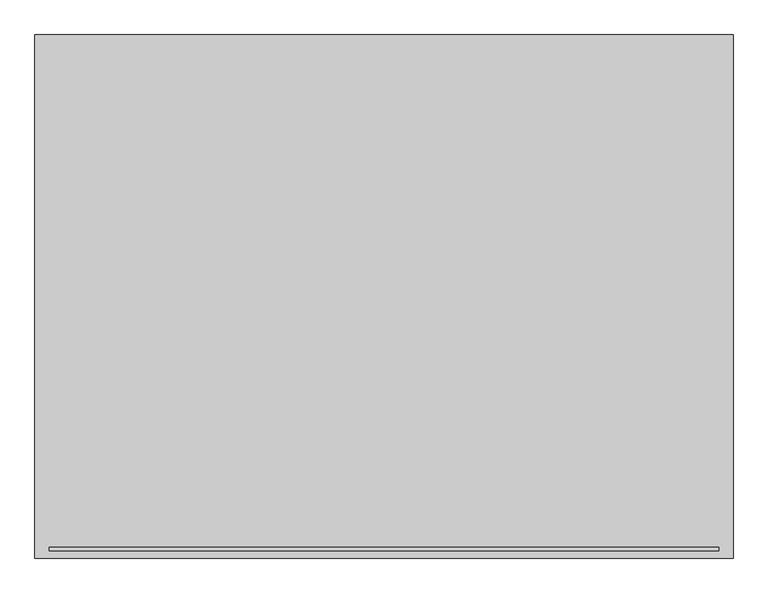
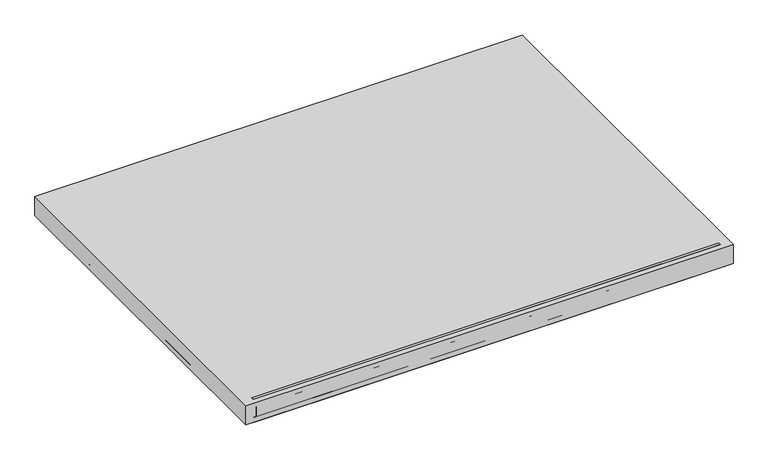
"""IFC4 building model written with IfcOpenShell, lengths in millimetres: proxy geometry, F3050 - Whiteboard, Dry Erase : F3050 - Whiteboard, Dry Erase."""

import ifcopenshell
import ifcopenshell.guid

model = None  # the IFC model being written
_history = None  # IfcOwnerHistory: only IFC2X3 demands one
_inside = {}  # id of a spatial element -> (the spatial element, [elements in it])
_under = {}  # id of a project, library or spatial element -> (it, [spatial elements below it])
_declared = {}  # id of a project -> (the project, [libraries it declares])
_typed = {}  # id of a type object -> (the type object, [elements of that type])
_made_of = {}  # id of a material, layer set ... -> (it, [elements and type objects made of it])


def new_model(schema):
    """Start an empty IFC model of exactly this schema.

    Asked for "IFC4X3", IfcOpenShell would pick the latest addendum, in which some entities
    have other attributes; the version numbers below select the first issue.
    IFC2X3 requires an IfcOwnerHistory on every rooted entity: one is made here for all.
    """
    global model, _history
    if schema == "IFC4X3":
        model = ifcopenshell.file(schema_version=(4, 3, 0, 0))
    else:
        model = ifcopenshell.file(schema=schema)
    _inside.clear()
    _under.clear()
    _declared.clear()
    _typed.clear()
    _made_of.clear()
    _history = None
    if model.schema == "IFC2X3":
        org = make("IfcOrganization", Name="unknown")
        user = make(
            "IfcPersonAndOrganization",
            ThePerson=make("IfcPerson", FamilyName="unknown"),
            TheOrganization=org,
        )
        app = make(
            "IfcApplication",
            ApplicationDeveloper=org,
            Version="unknown",
            ApplicationFullName="unknown",
            ApplicationIdentifier="unknown",
        )
        _history = make(
            "IfcOwnerHistory",
            OwningUser=user,
            OwningApplication=app,
            ChangeAction="ADDED",
            CreationDate=0,
        )
    return model


def make(cls, **values):
    """One entity of the class cls with the attributes given. An attribute that is None is left unset."""
    return model.create_entity(
        cls, **{name: value for name, value in values.items() if value is not None}
    )


def rooted(cls, **values):
    """An entity with a GlobalId (a new one), such as an element, a storey or a relation."""
    return make(cls, GlobalId=ifcopenshell.guid.new(), OwnerHistory=_history, **values)


def si_unit(unit_type, name, prefix=None):
    """IfcSIUnit, for example si_unit("LENGTHUNIT", "METRE", prefix="MILLI")."""
    return make("IfcSIUnit", UnitType=unit_type, Prefix=prefix, Name=name)


def assignment(units):
    """IfcUnitAssignment: the units of a project."""
    return None if units is None else make("IfcUnitAssignment", Units=units)


def point(xyz):
    """IfcCartesianPoint."""
    return None if xyz is None else make("IfcCartesianPoint", Coordinates=xyz)


def direction(xyz):
    """IfcDirection."""
    return None if xyz is None else make("IfcDirection", DirectionRatios=xyz)


def frame(location, z_axis=None, x_axis=None):
    """IfcAxis2Placement3D, a coordinate frame: its origin and axes. An axis left out is left unset."""
    return make(
        "IfcAxis2Placement3D",
        Location=point(location),
        Axis=direction(z_axis),
        RefDirection=direction(x_axis),
    )


def frame_2d(location, x_axis=None):
    """IfcAxis2Placement2D, a coordinate frame in the plane: its origin and x axis."""
    return make(
        "IfcAxis2Placement2D", Location=point(location), RefDirection=direction(x_axis)
    )


def origin():
    """The frame at (0, 0, 0) with its axes left unset."""
    return frame((0.0, 0.0, 0.0))


def origin_with_axes():
    """The frame at (0, 0, 0) with the z axis (0, 0, 1) and the x axis (1, 0, 0) written out."""
    return frame((0.0, 0.0, 0.0), z_axis=(0.0, 0.0, 1.0), x_axis=(1.0, 0.0, 0.0))


def place(relative_to, where):
    """IfcLocalPlacement: puts the frame where relative to a parent placement (None: the world)."""
    return make(
        "IfcLocalPlacement", PlacementRelTo=relative_to, RelativePlacement=where
    )


def context(
    kind, dimensions, precision=None, world=None, true_north=None, identifier=None
):
    """IfcGeometricRepresentationContext, for example the 3D "Model" context."""
    return make(
        "IfcGeometricRepresentationContext",
        ContextIdentifier=identifier,
        ContextType=kind,
        CoordinateSpaceDimension=dimensions,
        Precision=precision,
        WorldCoordinateSystem=world,
        TrueNorth=true_north,
    )


def project(units=None, contexts=None):
    """IfcProject with its units and contexts."""
    return rooted(
        "IfcProject",
        Name="project",
        RepresentationContexts=contexts,
        UnitsInContext=assignment(units),
    )


def spatial(cls, under=None, at=None, **own):
    """A site, building, storey or space (cls), placed at a placement, below another one or the project."""
    s = rooted(cls, ObjectPlacement=at, **own)
    if under is not None:
        _under.setdefault(under.id(), (under, []))[1].append(s)
    return s


def polyline(points):
    """IfcPolyline through the points."""
    return make("IfcPolyline", Points=[point(p) for p in points])


def circle_curve(where, radius):
    """IfcCircle in the frame where."""
    return make("IfcCircle", Position=where, Radius=radius)


def trimmed(basis, trim1, trim2, sense, master):
    """IfcTrimmedCurve: the piece of a basis curve between two trims."""
    return make(
        "IfcTrimmedCurve",
        BasisCurve=basis,
        Trim1=trim1,
        Trim2=trim2,
        SenseAgreement=sense,
        MasterRepresentation=master,
    )


def segment(curve, same_sense, transition):
    """IfcCompositeCurveSegment."""
    return make(
        "IfcCompositeCurveSegment",
        Transition=transition,
        SameSense=same_sense,
        ParentCurve=curve,
    )


def composite_curve(segments, self_intersect=None):
    """IfcCompositeCurve: segments joined end to end."""
    return make("IfcCompositeCurve", Segments=segments, SelfIntersect=self_intersect)


def outline(outer, holes=None, kind="AREA"):
    """IfcArbitraryClosedProfileDef: a profile drawn as a closed curve; with holes, ...WithVoids."""
    if holes is None:
        return make("IfcArbitraryClosedProfileDef", ProfileType=kind, OuterCurve=outer)
    return make(
        "IfcArbitraryProfileDefWithVoids",
        ProfileType=kind,
        OuterCurve=outer,
        InnerCurves=holes,
    )


def extrude(swept, where, along, depth):
    """IfcExtrudedAreaSolid: the profile swept, set in the frame where, extruded along a direction by depth."""
    return make(
        "IfcExtrudedAreaSolid",
        SweptArea=swept,
        Position=where,
        ExtrudedDirection=direction(along),
        Depth=depth,
    )


def shape(context_of_items, identifier, shape_type, items):
    """IfcShapeRepresentation: the items that make up one representation, for example the "Body"."""
    return make(
        "IfcShapeRepresentation",
        ContextOfItems=context_of_items,
        RepresentationIdentifier=identifier,
        RepresentationType=shape_type,
        Items=items,
    )


def source(mapping_origin, context_of_items, identifier, shape_type, items):
    """IfcRepresentationMap: a shape defined once, which mapped items show again and again."""
    return make(
        "IfcRepresentationMap",
        MappingOrigin=mapping_origin,
        MappedRepresentation=shape(context_of_items, identifier, shape_type, items),
    )


def transform(
    local_origin,
    x_axis=None,
    y_axis=None,
    z_axis=None,
    scale=None,
    scale2=None,
    scale3=None,
    uniform=True,
):
    """IfcCartesianTransformationOperator3D, or its non-uniform kind. x_axis, y_axis, z_axis: its Axis1, 2, 3."""
    if uniform:
        return make(
            "IfcCartesianTransformationOperator3D",
            Axis1=direction(x_axis),
            Axis2=direction(y_axis),
            LocalOrigin=point(local_origin),
            Scale=scale,
            Axis3=direction(z_axis),
        )
    return make(
        "IfcCartesianTransformationOperator3DnonUniform",
        Axis1=direction(x_axis),
        Axis2=direction(y_axis),
        LocalOrigin=point(local_origin),
        Scale=scale,
        Axis3=direction(z_axis),
        Scale2=scale2,
        Scale3=scale3,
    )


def mapped(mapping_source, mapping_target):
    """IfcMappedItem: shows the shape of a source again, moved by a transform."""
    return make(
        "IfcMappedItem", MappingSource=mapping_source, MappingTarget=mapping_target
    )


def made_of(thing, what):
    """Note that an element or type object is made of a material, layer set ...; save() writes the relation."""
    if what is not None:
        _made_of.setdefault(what.id(), (what, []))[1].append(thing)
    return thing


def element(
    cls,
    number,
    at=None,
    inside=None,
    cuts=None,
    type_object=None,
    material=None,
    context=None,
    identifier="Body",
    shape_type=None,
    held_by="IfcProductDefinitionShape",
    body=None,
    shapes=None,
    **own,
):
    """One element of the class cls, such as IfcWall. Its Tag is "e" and its number.

    at: its placement. inside: the storey or other place that contains it. cuts: it is an
    opening in that element (IfcRelVoidsElement). A single representation is given by context,
    identifier, shape_type and body (its items); several are given by shapes. held_by: the class
    of the entity that holds the representations. save() writes the other relations.
    """
    e = rooted(cls, Tag="e%d" % number, ObjectPlacement=at, **own)
    if body is not None:
        shapes = [shape(context, identifier, shape_type, body)]
    if shapes is not None:
        e.Representation = make(held_by, Representations=shapes)
    if inside is not None:
        _inside.setdefault(inside.id(), (inside, []))[1].append(e)
    if cuts is not None:
        rooted(
            "IfcRelVoidsElement", RelatingBuildingElement=cuts, RelatedOpeningElement=e
        )
    if type_object is not None:
        _typed.setdefault(type_object.id(), (type_object, []))[1].append(e)
    return made_of(e, material)


def aggregate(whole, parts):
    """IfcRelAggregates: a whole, such as a stair, and the parts it consists of."""
    return rooted("IfcRelAggregates", RelatingObject=whole, RelatedObjects=parts)


def save(model, path):
    """Write the relations noted so far, then the file.

    IfcRelAggregates (storeys below a building ...), IfcRelContainedInSpatialStructure (elements
    in a storey), IfcRelDefinesByType, IfcRelAssociatesMaterial and IfcRelDeclares: one each for
    every whole, place, type object, material and project.
    """
    for whole, parts in _under.values():
        aggregate(whole, parts)
    for where, things in _inside.values():
        rooted(
            "IfcRelContainedInSpatialStructure",
            RelatedElements=things,
            RelatingStructure=where,
        )
    for kind, things in _typed.values():
        rooted("IfcRelDefinesByType", RelatedObjects=things, RelatingType=kind)
    for what, things in _made_of.values():
        rooted("IfcRelAssociatesMaterial", RelatedObjects=things, RelatingMaterial=what)
    for by, libraries in _declared.values():
        rooted("IfcRelDeclares", RelatingContext=by, RelatedDefinitions=libraries)
    model.write(path)


def specialty_equipment_d43642da(model_context):
    return source(origin(), model_context, "Body", "SweptSolid", [
        extrude(outline(polyline([(609.6, 457.2), (609.6, -457.2), (-609.6, -457.2), (-609.6, 457.2), (609.6, 457.2)])), origin_with_axes(), (0.0, 0.0, 1.0), 50.8),
        extrude(outline(composite_curve([segment(trimmed(circle_curve(frame_2d((571.5, -419.1)), 12.7), [point((584.2, -419.1))], [point((571.5, -431.8))], False, "CARTESIAN"), True, "CONTINUOUS"), segment(polyline([(571.5, -431.8), (-571.5, -431.8)]), True, "CONTINUOUS"), segment(trimmed(circle_curve(frame_2d((-571.5, -419.1)), 12.7), [point((-571.5, -431.8))], [point((-584.2, -419.1))], False, "CARTESIAN"), True, "CONTINUOUS"), segment(polyline([(-584.2, -419.1), (-584.2, 419.1)]), True, "CONTINUOUS"), segment(trimmed(circle_curve(frame_2d((-571.5, 419.1)), 12.7), [point((-584.2, 419.1))], [point((-571.5, 431.8))], False, "CARTESIAN"), True, "CONTINUOUS"), segment(polyline([(-571.5, 431.8), (571.5, 431.8)]), True, "CONTINUOUS"), segment(trimmed(circle_curve(frame_2d((571.5, 419.1)), 12.7), [point((571.5, 431.8))], [point((584.2, 419.1))], False, "CARTESIAN"), True, "CONTINUOUS"), segment(polyline([(584.2, 419.1), (584.2, -419.1)]), True, "CONTINUOUS")], self_intersect=False)), origin_with_axes(), (0.0, 0.0, 1.0), 6.6972656),
        extrude(outline(polyline([(-438.15, 51.4978879), (-438.15, 13.3978879), (-457.2, 13.3978879), (-457.2, 38.7978879), (-450.85, 38.7978879), (-450.85, 45.1478879), (-444.5, 45.1478879), (-444.5, 51.4978879), (-438.15, 51.4978879)])), frame((-584.2, 0.0, 0.0), z_axis=(1.0, 0.0, 0.0), x_axis=(0.0, 1.0, 0.0)), (0.0, 0.0, 1.0), 1168.4),
        extrude(outline(composite_curve([segment(trimmed(circle_curve(frame_2d((584.2, 431.8)), 25.4), [point((584.2, 457.2))], [point((609.6, 431.8))], False, "CARTESIAN"), True, "CONTINUOUS"), segment(polyline([(609.6, 431.8), (609.6, -431.8)]), True, "CONTINUOUS"), segment(trimmed(circle_curve(frame_2d((584.2, -431.8)), 25.4), [point((609.6, -431.8))], [point((584.2, -457.2))], False, "CARTESIAN"), True, "CONTINUOUS"), segment(polyline([(584.2, -457.2), (-589.1477625, -457.2)]), True, "CONTINUOUS"), segment(trimmed(circle_curve(frame_2d((-589.1477625, -436.7477625)), 20.4522375), [point((-589.1477625, -457.2))], [point((-609.6, -436.7477625))], False, "CARTESIAN"), True, "CONTINUOUS"), segment(polyline([(-609.6, -436.7477625), (-609.6, 436.7477625)]), True, "CONTINUOUS"), segment(trimmed(circle_curve(frame_2d((-589.1477625, 436.7477625)), 20.4522375), [point((-609.6, 436.7477625))], [point((-589.1477625, 457.2))], False, "CARTESIAN"), True, "CONTINUOUS"), segment(polyline([(-589.1477625, 457.2), (584.2, 457.2)]), True, "CONTINUOUS")], self_intersect=False), holes=[composite_curve([segment(polyline([(571.5, 431.8), (-571.5, 431.8)]), True, "CONTINUOUS"), segment(trimmed(circle_curve(frame_2d((-571.5, 419.1)), 12.7), [point((-571.5, 431.8))], [point((-584.2, 419.1))], True, "CARTESIAN"), True, "CONTINUOUS"), segment(polyline([(-584.2, 419.1), (-584.2, -419.1)]), True, "CONTINUOUS"), segment(trimmed(circle_curve(frame_2d((-571.5, -419.1)), 12.7), [point((-584.2, -419.1))], [point((-571.5, -431.8))], True, "CARTESIAN"), True, "CONTINUOUS"), segment(polyline([(-571.5, -431.8), (571.5, -431.8)]), True, "CONTINUOUS"), segment(trimmed(circle_curve(frame_2d((571.5, -419.1)), 12.7), [point((571.5, -431.8))], [point((584.2, -419.1))], True, "CARTESIAN"), True, "CONTINUOUS"), segment(polyline([(584.2, -419.1), (584.2, 419.1)]), True, "CONTINUOUS"), segment(trimmed(circle_curve(frame_2d((571.5, 419.1)), 12.7), [point((584.2, 419.1))], [point((571.5, 431.8))], True, "CARTESIAN"), True, "CONTINUOUS")], self_intersect=False)]), origin_with_axes(), (0.0, 0.0, 1.0), 13.3978879),
    ])


if __name__ == "__main__":
    model = new_model("IFC4")
    model_context = context("Model", 3, world=origin())
    ifc_project = project(units=[si_unit("LENGTHUNIT", "METRE", prefix="MILLI")], contexts=[model_context])
    site = spatial("IfcSite", under=ifc_project)
    building = spatial("IfcBuilding", under=site)
    placement = place(None, origin())
    specialty_equipment_shape = specialty_equipment_d43642da(model_context)
    element("IfcBuildingElementProxy", 1, Name="F3050 - Whiteboard, Dry Erase : F3050 - Whiteboard, Dry Erase", ObjectType="F3050 - Whiteboard, Dry Erase : F3050 - Whiteboard, Dry Erase", at=placement, inside=building, context=model_context, shape_type="MappedRepresentation", body=[
        mapped(specialty_equipment_shape, transform((0.0, 0.0, 0.0), x_axis=(1.0, 0.0, 0.0), y_axis=(0.0, 1.0, 0.0), z_axis=(0.0, 0.0, 1.0))),
    ])
    save(model, "model.ifc")

# Revit data of these elements
# Type "F3050 - Whiteboard, Dry Erase : F3050 - Whiteboard, Dry Erase"
#   Watts2 = "0"
#   Watts1 = "0"
#   Unit_Issue = "EA"
#   UTIL_6_Misc = "-"
#   UTIL_5_NonMedGas = "-"
#   UTIL_4_MiscGas = "-"
#   UTIL_3_MedGas = "-"
#   UTIL_2_Elec = "-"
#   UTIL_1_WaterDrain = "-"
#   Nomenclature = "Whiteboard, Dry Erase"
#   NSN = "7110"
#   Location [instance default] = ""
#   JSN = "F3050"
#   Fund_Source_VA = "-"
#   Fund_Source_Navy = "-"
#   Fund_Source_Army = "-"
#   Fund_Source_AF = "-"
#   ELEC_Volts2 = "0"
#   ELEC_Volts1 = "0"
#   ELEC_Phase2 = "0"
#   ELEC_Phase1 = "0"
#   ELEC_HertzSwitch = "0"
#   ELEC_HertzDependent = "0"
#   ELEC_Hertz = "0"
#   ELEC_Amps2 = "0"
#   ELEC_Amps1 = "0"
#   DetailDescription = "Whiteboard unit, approximately 36\" H x 48\" W consisting of a white porcelain enamel writing surface with an attached chalk tray. Magnetic surface available. Image can be easily removed with a standard chalkboard eraser. For use with water color pens. Unit is ready to hang."
#   CAT_VA = "A"
#   CAT_Navy = "A"
#   CAT_IHS = "-"
#   CAT_Army = "A"
#   CAT_AF = "A"
#   BTUperhour = "0"
#   Weight_IP = 30
#   Default Elevation = 5' - 0"
#   DIM_Width_IP = 4' - 0"
#   DIM_Height_IP = 3' - 0"
#   DIM_Depth_IP = 0' - 2"
# Element 1 (IfcBuildingElementProxy, "F3050 - Whiteboard, Dry Erase : F3050 - Whiteboard, Dry Erase")
#   Location = "ORGS1"
#   Materials on its faces: "White Plastic", "EquipSpace"
# Materials
#   "White Plastic": class "Unassigned", colour RGB 247 247 247, transparency 0, Comments = "Rendering appearance not upgraded "
#   "EquipSpace": class "Unassigned", colour RGB 221 217 195, transparency 0.5
